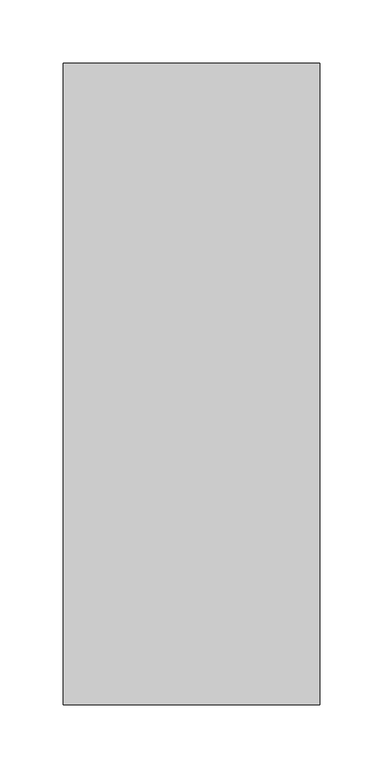
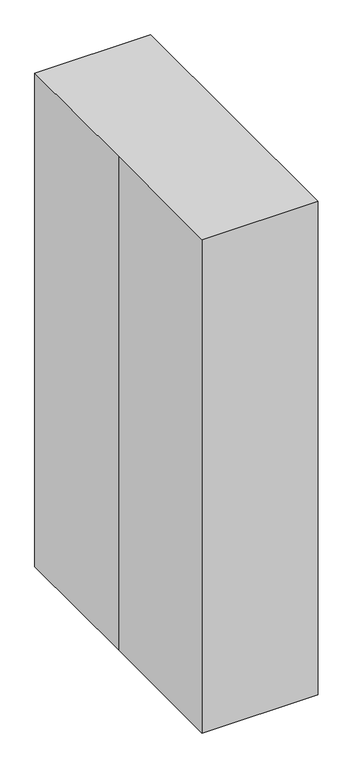
"""IFC4 building model written with IfcOpenShell, lengths in millimetres: proxy geometry, P1150 - Valve, Rinse, Bedpan, With Disinfectant Injector : P1150 - Valve, Rinse, Bedpan, With Disinfectant Injector."""

import ifcopenshell
import ifcopenshell.guid

model = None  # the IFC model being written
_history = None  # IfcOwnerHistory: only IFC2X3 demands one
_inside = {}  # id of a spatial element -> (the spatial element, [elements in it])
_under = {}  # id of a project, library or spatial element -> (it, [spatial elements below it])
_declared = {}  # id of a project -> (the project, [libraries it declares])
_typed = {}  # id of a type object -> (the type object, [elements of that type])
_made_of = {}  # id of a material, layer set ... -> (it, [elements and type objects made of it])


def new_model(schema):
    """Start an empty IFC model of exactly this schema.

    Asked for "IFC4X3", IfcOpenShell would pick the latest addendum, in which some entities
    have other attributes; the version numbers below select the first issue.
    IFC2X3 requires an IfcOwnerHistory on every rooted entity: one is made here for all.
    """
    global model, _history
    if schema == "IFC4X3":
        model = ifcopenshell.file(schema_version=(4, 3, 0, 0))
    else:
        model = ifcopenshell.file(schema=schema)
    _inside.clear()
    _under.clear()
    _declared.clear()
    _typed.clear()
    _made_of.clear()
    _history = None
    if model.schema == "IFC2X3":
        org = make("IfcOrganization", Name="unknown")
        user = make(
            "IfcPersonAndOrganization",
            ThePerson=make("IfcPerson", FamilyName="unknown"),
            TheOrganization=org,
        )
        app = make(
            "IfcApplication",
            ApplicationDeveloper=org,
            Version="unknown",
            ApplicationFullName="unknown",
            ApplicationIdentifier="unknown",
        )
        _history = make(
            "IfcOwnerHistory",
            OwningUser=user,
            OwningApplication=app,
            ChangeAction="ADDED",
            CreationDate=0,
        )
    return model


def make(cls, **values):
    """One entity of the class cls with the attributes given. An attribute that is None is left unset."""
    return model.create_entity(
        cls, **{name: value for name, value in values.items() if value is not None}
    )


def rooted(cls, **values):
    """An entity with a GlobalId (a new one), such as an element, a storey or a relation."""
    return make(cls, GlobalId=ifcopenshell.guid.new(), OwnerHistory=_history, **values)


def si_unit(unit_type, name, prefix=None):
    """IfcSIUnit, for example si_unit("LENGTHUNIT", "METRE", prefix="MILLI")."""
    return make("IfcSIUnit", UnitType=unit_type, Prefix=prefix, Name=name)


def assignment(units):
    """IfcUnitAssignment: the units of a project."""
    return None if units is None else make("IfcUnitAssignment", Units=units)


def point(xyz):
    """IfcCartesianPoint."""
    return None if xyz is None else make("IfcCartesianPoint", Coordinates=xyz)


def direction(xyz):
    """IfcDirection."""
    return None if xyz is None else make("IfcDirection", DirectionRatios=xyz)


def frame(location, z_axis=None, x_axis=None):
    """IfcAxis2Placement3D, a coordinate frame: its origin and axes. An axis left out is left unset."""
    return make(
        "IfcAxis2Placement3D",
        Location=point(location),
        Axis=direction(z_axis),
        RefDirection=direction(x_axis),
    )


def frame_2d(location, x_axis=None):
    """IfcAxis2Placement2D, a coordinate frame in the plane: its origin and x axis."""
    return make(
        "IfcAxis2Placement2D", Location=point(location), RefDirection=direction(x_axis)
    )


def origin():
    """The frame at (0, 0, 0) with its axes left unset."""
    return frame((0.0, 0.0, 0.0))


def origin_with_axes():
    """The frame at (0, 0, 0) with the z axis (0, 0, 1) and the x axis (1, 0, 0) written out."""
    return frame((0.0, 0.0, 0.0), z_axis=(0.0, 0.0, 1.0), x_axis=(1.0, 0.0, 0.0))


def origin_2d():
    """The frame at (0, 0) in the plane with its x axis left unset."""
    return frame_2d((0.0, 0.0))


def place(relative_to, where):
    """IfcLocalPlacement: puts the frame where relative to a parent placement (None: the world)."""
    return make(
        "IfcLocalPlacement", PlacementRelTo=relative_to, RelativePlacement=where
    )


def context(
    kind, dimensions, precision=None, world=None, true_north=None, identifier=None
):
    """IfcGeometricRepresentationContext, for example the 3D "Model" context."""
    return make(
        "IfcGeometricRepresentationContext",
        ContextIdentifier=identifier,
        ContextType=kind,
        CoordinateSpaceDimension=dimensions,
        Precision=precision,
        WorldCoordinateSystem=world,
        TrueNorth=true_north,
    )


def project(units=None, contexts=None):
    """IfcProject with its units and contexts."""
    return rooted(
        "IfcProject",
        Name="project",
        RepresentationContexts=contexts,
        UnitsInContext=assignment(units),
    )


def spatial(cls, under=None, at=None, **own):
    """A site, building, storey or space (cls), placed at a placement, below another one or the project."""
    s = rooted(cls, ObjectPlacement=at, **own)
    if under is not None:
        _under.setdefault(under.id(), (under, []))[1].append(s)
    return s


def polyline(points):
    """IfcPolyline through the points."""
    return make("IfcPolyline", Points=[point(p) for p in points])


def circle_curve(where, radius):
    """IfcCircle in the frame where."""
    return make("IfcCircle", Position=where, Radius=radius)


def trimmed(basis, trim1, trim2, sense, master):
    """IfcTrimmedCurve: the piece of a basis curve between two trims."""
    return make(
        "IfcTrimmedCurve",
        BasisCurve=basis,
        Trim1=trim1,
        Trim2=trim2,
        SenseAgreement=sense,
        MasterRepresentation=master,
    )


def segment(curve, same_sense, transition):
    """IfcCompositeCurveSegment."""
    return make(
        "IfcCompositeCurveSegment",
        Transition=transition,
        SameSense=same_sense,
        ParentCurve=curve,
    )


def composite_curve(segments, self_intersect=None):
    """IfcCompositeCurve: segments joined end to end."""
    return make("IfcCompositeCurve", Segments=segments, SelfIntersect=self_intersect)


def outline(outer, holes=None, kind="AREA"):
    """IfcArbitraryClosedProfileDef: a profile drawn as a closed curve; with holes, ...WithVoids."""
    if holes is None:
        return make("IfcArbitraryClosedProfileDef", ProfileType=kind, OuterCurve=outer)
    return make(
        "IfcArbitraryProfileDefWithVoids",
        ProfileType=kind,
        OuterCurve=outer,
        InnerCurves=holes,
    )


def extrude(swept, where, along, depth):
    """IfcExtrudedAreaSolid: the profile swept, set in the frame where, extruded along a direction by depth."""
    return make(
        "IfcExtrudedAreaSolid",
        SweptArea=swept,
        Position=where,
        ExtrudedDirection=direction(along),
        Depth=depth,
    )


def shape(context_of_items, identifier, shape_type, items):
    """IfcShapeRepresentation: the items that make up one representation, for example the "Body"."""
    return make(
        "IfcShapeRepresentation",
        ContextOfItems=context_of_items,
        RepresentationIdentifier=identifier,
        RepresentationType=shape_type,
        Items=items,
    )


def source(mapping_origin, context_of_items, identifier, shape_type, items):
    """IfcRepresentationMap: a shape defined once, which mapped items show again and again."""
    return make(
        "IfcRepresentationMap",
        MappingOrigin=mapping_origin,
        MappedRepresentation=shape(context_of_items, identifier, shape_type, items),
    )


def transform(
    local_origin,
    x_axis=None,
    y_axis=None,
    z_axis=None,
    scale=None,
    scale2=None,
    scale3=None,
    uniform=True,
):
    """IfcCartesianTransformationOperator3D, or its non-uniform kind. x_axis, y_axis, z_axis: its Axis1, 2, 3."""
    if uniform:
        return make(
            "IfcCartesianTransformationOperator3D",
            Axis1=direction(x_axis),
            Axis2=direction(y_axis),
            LocalOrigin=point(local_origin),
            Scale=scale,
            Axis3=direction(z_axis),
        )
    return make(
        "IfcCartesianTransformationOperator3DnonUniform",
        Axis1=direction(x_axis),
        Axis2=direction(y_axis),
        LocalOrigin=point(local_origin),
        Scale=scale,
        Axis3=direction(z_axis),
        Scale2=scale2,
        Scale3=scale3,
    )


def mapped(mapping_source, mapping_target):
    """IfcMappedItem: shows the shape of a source again, moved by a transform."""
    return make(
        "IfcMappedItem", MappingSource=mapping_source, MappingTarget=mapping_target
    )


def made_of(thing, what):
    """Note that an element or type object is made of a material, layer set ...; save() writes the relation."""
    if what is not None:
        _made_of.setdefault(what.id(), (what, []))[1].append(thing)
    return thing


def element(
    cls,
    number,
    at=None,
    inside=None,
    cuts=None,
    type_object=None,
    material=None,
    context=None,
    identifier="Body",
    shape_type=None,
    held_by="IfcProductDefinitionShape",
    body=None,
    shapes=None,
    **own,
):
    """One element of the class cls, such as IfcWall. Its Tag is "e" and its number.

    at: its placement. inside: the storey or other place that contains it. cuts: it is an
    opening in that element (IfcRelVoidsElement). A single representation is given by context,
    identifier, shape_type and body (its items); several are given by shapes. held_by: the class
    of the entity that holds the representations. save() writes the other relations.
    """
    e = rooted(cls, Tag="e%d" % number, ObjectPlacement=at, **own)
    if body is not None:
        shapes = [shape(context, identifier, shape_type, body)]
    if shapes is not None:
        e.Representation = make(held_by, Representations=shapes)
    if inside is not None:
        _inside.setdefault(inside.id(), (inside, []))[1].append(e)
    if cuts is not None:
        rooted(
            "IfcRelVoidsElement", RelatingBuildingElement=cuts, RelatedOpeningElement=e
        )
    if type_object is not None:
        _typed.setdefault(type_object.id(), (type_object, []))[1].append(e)
    return made_of(e, material)


def aggregate(whole, parts):
    """IfcRelAggregates: a whole, such as a stair, and the parts it consists of."""
    return rooted("IfcRelAggregates", RelatingObject=whole, RelatedObjects=parts)


def save(model, path):
    """Write the relations noted so far, then the file.

    IfcRelAggregates (storeys below a building ...), IfcRelContainedInSpatialStructure (elements
    in a storey), IfcRelDefinesByType, IfcRelAssociatesMaterial and IfcRelDeclares: one each for
    every whole, place, type object, material and project.
    """
    for whole, parts in _under.values():
        aggregate(whole, parts)
    for where, things in _inside.values():
        rooted(
            "IfcRelContainedInSpatialStructure",
            RelatedElements=things,
            RelatingStructure=where,
        )
    for kind, things in _typed.values():
        rooted("IfcRelDefinesByType", RelatedObjects=things, RelatingType=kind)
    for what, things in _made_of.values():
        rooted("IfcRelAssociatesMaterial", RelatedObjects=things, RelatingMaterial=what)
    for by, libraries in _declared.values():
        rooted("IfcRelDeclares", RelatingContext=by, RelatedDefinitions=libraries)
    model.write(path)


def specialty_equipment_cf81bb52(model_context):
    return source(origin(), model_context, "Body", "SweptSolid", [
        extrude(outline(composite_curve([segment(trimmed(circle_curve(frame_2d((0.0, 400.05)), 19.05), [point((-19.05, 400.05))], [point((19.05, 400.05))], False, "CARTESIAN"), True, "CONTINUOUS"), segment(trimmed(circle_curve(frame_2d((0.0, 400.05)), 19.05), [point((19.05, 400.05))], [point((-19.05, 400.05))], False, "CARTESIAN"), True, "CONTINUOUS")], self_intersect=False)), frame((26.9875, 0.0, 0.0), z_axis=(1.0, 0.0, 0.0), x_axis=(0.0, 1.0, 0.0)), (0.0, 0.0, 1.0), 25.4),
        extrude(outline(composite_curve([segment(trimmed(circle_curve(frame_2d((50.8, 39.6875)), 19.05), [point((50.8, 20.6375))], [point((50.8, 58.7375))], False, "CARTESIAN"), True, "CONTINUOUS"), segment(trimmed(circle_curve(frame_2d((50.8, 39.6875)), 19.05), [point((50.8, 58.7375))], [point((50.8, 20.6375))], False, "CARTESIAN"), True, "CONTINUOUS")], self_intersect=False)), frame((0.0, -25.4, 0.0), z_axis=(0.0, 1.0, 0.0), x_axis=(0.0, 0.0, 1.0)), (0.0, 0.0, 1.0), 50.8),
        extrude(outline(composite_curve([segment(trimmed(circle_curve(frame_2d((39.6875, 0.0)), 6.35), [point((33.3375, 0.0))], [point((46.0375, 0.0))], False, "CARTESIAN"), True, "CONTINUOUS"), segment(trimmed(circle_curve(frame_2d((39.6875, 0.0)), 6.35), [point((46.0375, 0.0))], [point((33.3375, 0.0))], False, "CARTESIAN"), True, "CONTINUOUS")], self_intersect=False)), frame((0.0, 0.0, 50.8), z_axis=(0.0, 0.0, 1.0), x_axis=(1.0, 0.0, 0.0)), (0.0, 0.0, 1.0), 349.25),
        extrude(outline(composite_curve([segment(trimmed(circle_curve(origin_2d(), 31.75), [point((-31.75, 0.0))], [point((31.75, 0.0))], False, "CARTESIAN"), True, "CONTINUOUS"), segment(trimmed(circle_curve(origin_2d(), 31.75), [point((31.75, 0.0))], [point((-31.75, 0.0))], False, "CARTESIAN"), True, "CONTINUOUS")], self_intersect=False), holes=[composite_curve([segment(trimmed(circle_curve(origin_2d(), 25.4), [point((-25.4, 0.0))], [point((25.4, 0.0))], True, "CARTESIAN"), True, "CONTINUOUS"), segment(trimmed(circle_curve(origin_2d(), 25.4), [point((25.4, 0.0))], [point((-25.4, 0.0))], True, "CARTESIAN"), True, "CONTINUOUS")], self_intersect=False)]), frame((0.0, 0.0, 25.4), z_axis=(0.0, 0.0, 1.0), x_axis=(1.0, 0.0, 0.0)), (0.0, 0.0, 1.0), 50.8),
        extrude(outline(polyline([(-101.6, 254.0), (101.6, 254.0), (101.6, -254.0), (-101.6, -254.0), (-101.6, 0.0), (-101.6, 254.0)])), origin_with_axes(), (0.0, 0.0, 1.0), 914.4),
    ])


if __name__ == "__main__":
    model = new_model("IFC4")
    model_context = context("Model", 3, world=origin())
    ifc_project = project(units=[si_unit("LENGTHUNIT", "METRE", prefix="MILLI")], contexts=[model_context])
    site = spatial("IfcSite", under=ifc_project)
    building = spatial("IfcBuilding", under=site)
    placement = place(None, origin())
    specialty_equipment_shape = specialty_equipment_cf81bb52(model_context)
    element("IfcBuildingElementProxy", 1, Name="P1150 - Valve, Rinse, Bedpan, With Disinfectant Injector : P1150 - Valve, Rinse, Bedpan, With Disinfectant Injector", ObjectType="P1150 - Valve, Rinse, Bedpan, With Disinfectant Injector : P1150 - Valve, Rinse, Bedpan, With Disinfectant Injector", at=placement, inside=building, context=model_context, shape_type="MappedRepresentation", body=[
        mapped(specialty_equipment_shape, transform((0.0, 0.0, 0.0), x_axis=(1.0, 0.0, 0.0), y_axis=(0.0, 1.0, 0.0), z_axis=(0.0, 0.0, 1.0))),
    ])
    save(model, "model.ifc")

# Revit data of these elements
# Type "P1150 - Valve, Rinse, Bedpan, With Disinfectant Injector : P1150 - Valve, Rinse, Bedpan, With Disinfectant Injector"
#   Watts2 = "0"
#   Watts1 = "0"
#   Unit_Issue = "EA"
#   UTIL_6_Misc = "-"
#   UTIL_5_NonMedGas = "-"
#   UTIL_4_MiscGas = "-"
#   UTIL_3_MedGas = "-"
#   UTIL_2_Elec = "-"
#   UTIL_1_WaterDrain = "J"
#   Nomenclature = "Valve, Rinse, Bedpan, With Disinfectant Injector"
#   NSN = "4510"
#   Location [instance default] = ""
#   JSN = "P1150"
#   Fund_Source_VA = "-"
#   Fund_Source_Navy = "-"
#   Fund_Source_Army = "-"
#   Fund_Source_AF = "-"
#   ELEC_Volts2 = "0"
#   ELEC_Volts1 = "0"
#   ELEC_Phase2 = "0"
#   ELEC_Phase1 = "0"
#   ELEC_HertzSwitch = "0"
#   ELEC_HertzDependent = "0"
#   ELEC_Hertz = "0"
#   ELEC_Amps2 = "0"
#   ELEC_Amps1 = "0"
#   DetailDescription = "Bedpan rinsing valve with deodorant/disinfectant spray. Unit is wall mounted above a water closet having an exposed flush valve. Flush water shall be available to rinse the pan with the balance used to flush the waste. Used in dirty utility rooms located in patient care areas throughout the hospital. Unit is used to flush and disinfect a dirty bedpan."
#   CAT_VA = "A"
#   CAT_Navy = "A"
#   CAT_IHS = "-"
#   CAT_Army = "A"
#   CAT_AF = "A"
#   BTUperhour = "0"
#   Weight_IP = 8
#   DIM_Width_IP = 0' - 8"
#   DIM_Height_IP = 3' - 0"
#   DIM_Depth_IP = 1' - 8"
# Element 1 (IfcBuildingElementProxy, "P1150 - Valve, Rinse, Bedpan, With Disinfectant Injector : P1150 - Valve, Rinse, Bedpan, With Disinfectant Injector")
#   Materials on its faces: "EquipSpace"
# Materials
#   "EquipSpace": class "Unassigned", colour RGB 221 217 195, transparency 0.5
